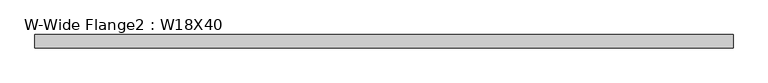
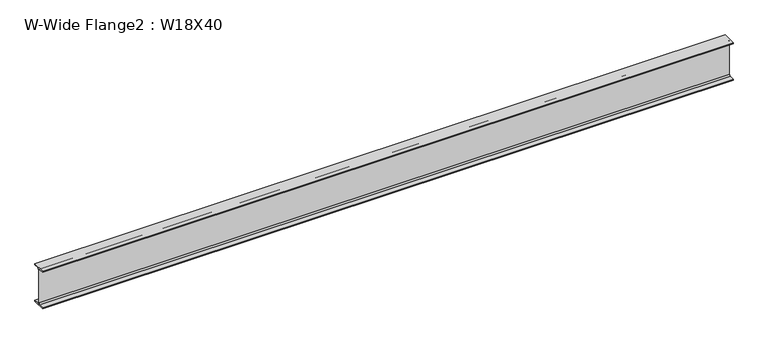
"""IFC4 building model written with IfcOpenShell, lengths in millimetres: beam geometry, W-Wide Flange2 : W18X40."""

from ifc_helpers import new_model, si_unit, point, frame, frame_2d, origin, place, context, project, spatial, polyline, circle_curve, trimmed, segment, composite_curve, outline, extrude, source, transform, mapped, element, save


def w_wide_flange2_w18x40_61f41169(model_context):
    return source(origin(), model_context, "Body", "SweptSolid", [
        extrude(outline(composite_curve([segment(polyline([(76.454, -213.995), (76.454, -227.33), (-76.454, -227.33), (-76.454, -213.995), (-20.828, -213.995)]), True, "CONTINUOUS"), segment(trimmed(circle_curve(frame_2d((-20.828, -197.1675)), 16.8275), [point((-20.828, -213.995))], [point((-4.0005, -197.1675))], True, "CARTESIAN"), True, "CONTINUOUS"), segment(polyline([(-4.0005, -197.1675), (-4.0005, 197.1675)]), True, "CONTINUOUS"), segment(trimmed(circle_curve(frame_2d((-20.828, 197.1675)), 16.8275), [point((-4.0005, 197.1675))], [point((-20.828, 213.995))], True, "CARTESIAN"), True, "CONTINUOUS"), segment(polyline([(-20.828, 213.995), (-76.454, 213.995), (-76.454, 227.33), (76.454, 227.33), (76.454, 213.995), (20.828, 213.995)]), True, "CONTINUOUS"), segment(trimmed(circle_curve(frame_2d((20.828, 197.1675)), 16.8275), [point((20.828, 213.995))], [point((4.0005, 197.1675))], True, "CARTESIAN"), True, "CONTINUOUS"), segment(polyline([(4.0005, 197.1675), (4.0005, -197.1675)]), True, "CONTINUOUS"), segment(trimmed(circle_curve(frame_2d((20.828, -197.1675)), 16.8275), [point((4.0005, -197.1675))], [point((20.828, -213.995))], True, "CARTESIAN"), True, "CONTINUOUS"), segment(polyline([(20.828, -213.995), (76.454, -213.995)]), True, "CONTINUOUS")], self_intersect=False)), frame((-3922.7125, 0.0, 0.0), z_axis=(1.0, 0.0, 0.0), x_axis=(0.0, 1.0, 0.0)), (0.0, 0.0, 1.0), 7902.575),
    ])


if __name__ == "__main__":
    model = new_model("IFC4")
    model_context = context("Model", 3, world=origin())
    ifc_project = project(units=[si_unit("LENGTHUNIT", "METRE", prefix="MILLI")], contexts=[model_context])
    site = spatial("IfcSite", under=ifc_project)
    building = spatial("IfcBuilding", under=site)
    placement = place(None, origin())
    w_wide_flange2_w18x40_shape = w_wide_flange2_w18x40_61f41169(model_context)
    element("IfcBeam", 1, ObjectType="W-Wide Flange2 : W18X40", at=placement, inside=building, context=model_context, shape_type="MappedRepresentation", body=[
        mapped(w_wide_flange2_w18x40_shape, transform((0.0, 0.0, 0.0), x_axis=(1.0, 0.0, 0.0), y_axis=(0.0, 1.0, 0.0), z_axis=(0.0, 0.0, 1.0))),
    ])
    save(model, "model.ifc")

# Revit data of these elements
# Type "W-Wide Flange2 : W18X40"
#   Assembly Code = "B10"
#   W = 40
#   Length [instance default] = 5' - 0"
#   bf = 0' - 6.02"
#   d = 1' - 5.9"
#   k = 0' - 1 3/16"
#   k2 = 0' - 0.6625"
#   tf = 0' - 0.525"
#   tw = 0' - 0.315"
#   A = 0.0819444 SF
#   Structural Material [instance default] = Steel ASTM A992
# Element 1 (IfcBeam, "W-Wide Flange2 : W18X40")
#   Materials on its faces: "Steel ASTM A992"
# Materials
#   "Steel ASTM A992": class "Metal", colour RGB 199 199 199, transparency 0, Description = "Structural steel 50ksi", Cost = 0
